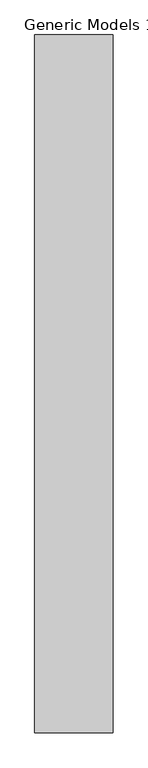
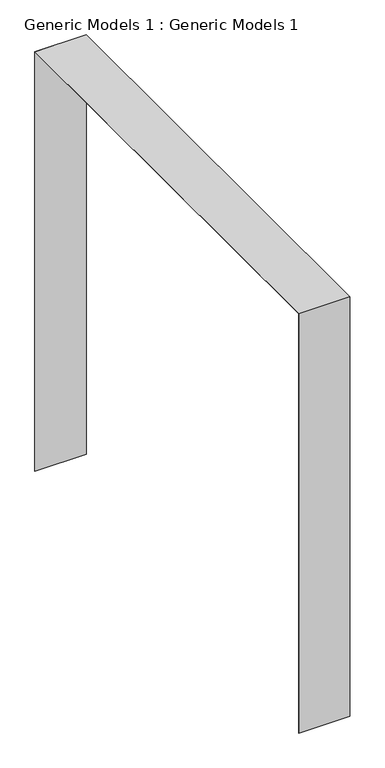
"""IFC4 building model written with IfcOpenShell, lengths in millimetres: proxy geometry, Generic Models 1 : Generic Models 1."""

import ifcopenshell
import ifcopenshell.guid

model = None  # the IFC model being written
_history = None  # IfcOwnerHistory: only IFC2X3 demands one
_inside = {}  # id of a spatial element -> (the spatial element, [elements in it])
_under = {}  # id of a project, library or spatial element -> (it, [spatial elements below it])
_declared = {}  # id of a project -> (the project, [libraries it declares])
_typed = {}  # id of a type object -> (the type object, [elements of that type])
_made_of = {}  # id of a material, layer set ... -> (it, [elements and type objects made of it])


def new_model(schema):
    """Start an empty IFC model of exactly this schema.

    Asked for "IFC4X3", IfcOpenShell would pick the latest addendum, in which some entities
    have other attributes; the version numbers below select the first issue.
    IFC2X3 requires an IfcOwnerHistory on every rooted entity: one is made here for all.
    """
    global model, _history
    if schema == "IFC4X3":
        model = ifcopenshell.file(schema_version=(4, 3, 0, 0))
    else:
        model = ifcopenshell.file(schema=schema)
    _inside.clear()
    _under.clear()
    _declared.clear()
    _typed.clear()
    _made_of.clear()
    _history = None
    if model.schema == "IFC2X3":
        org = make("IfcOrganization", Name="unknown")
        user = make(
            "IfcPersonAndOrganization",
            ThePerson=make("IfcPerson", FamilyName="unknown"),
            TheOrganization=org,
        )
        app = make(
            "IfcApplication",
            ApplicationDeveloper=org,
            Version="unknown",
            ApplicationFullName="unknown",
            ApplicationIdentifier="unknown",
        )
        _history = make(
            "IfcOwnerHistory",
            OwningUser=user,
            OwningApplication=app,
            ChangeAction="ADDED",
            CreationDate=0,
        )
    return model


def make(cls, **values):
    """One entity of the class cls with the attributes given. An attribute that is None is left unset."""
    return model.create_entity(
        cls, **{name: value for name, value in values.items() if value is not None}
    )


def rooted(cls, **values):
    """An entity with a GlobalId (a new one), such as an element, a storey or a relation."""
    return make(cls, GlobalId=ifcopenshell.guid.new(), OwnerHistory=_history, **values)


def si_unit(unit_type, name, prefix=None):
    """IfcSIUnit, for example si_unit("LENGTHUNIT", "METRE", prefix="MILLI")."""
    return make("IfcSIUnit", UnitType=unit_type, Prefix=prefix, Name=name)


def assignment(units):
    """IfcUnitAssignment: the units of a project."""
    return None if units is None else make("IfcUnitAssignment", Units=units)


def point(xyz):
    """IfcCartesianPoint."""
    return None if xyz is None else make("IfcCartesianPoint", Coordinates=xyz)


def direction(xyz):
    """IfcDirection."""
    return None if xyz is None else make("IfcDirection", DirectionRatios=xyz)


def frame(location, z_axis=None, x_axis=None):
    """IfcAxis2Placement3D, a coordinate frame: its origin and axes. An axis left out is left unset."""
    return make(
        "IfcAxis2Placement3D",
        Location=point(location),
        Axis=direction(z_axis),
        RefDirection=direction(x_axis),
    )


def origin():
    """The frame at (0, 0, 0) with its axes left unset."""
    return frame((0.0, 0.0, 0.0))


def place(relative_to, where):
    """IfcLocalPlacement: puts the frame where relative to a parent placement (None: the world)."""
    return make(
        "IfcLocalPlacement", PlacementRelTo=relative_to, RelativePlacement=where
    )


def context(
    kind, dimensions, precision=None, world=None, true_north=None, identifier=None
):
    """IfcGeometricRepresentationContext, for example the 3D "Model" context."""
    return make(
        "IfcGeometricRepresentationContext",
        ContextIdentifier=identifier,
        ContextType=kind,
        CoordinateSpaceDimension=dimensions,
        Precision=precision,
        WorldCoordinateSystem=world,
        TrueNorth=true_north,
    )


def project(units=None, contexts=None):
    """IfcProject with its units and contexts."""
    return rooted(
        "IfcProject",
        Name="project",
        RepresentationContexts=contexts,
        UnitsInContext=assignment(units),
    )


def spatial(cls, under=None, at=None, **own):
    """A site, building, storey or space (cls), placed at a placement, below another one or the project."""
    s = rooted(cls, ObjectPlacement=at, **own)
    if under is not None:
        _under.setdefault(under.id(), (under, []))[1].append(s)
    return s


def polyline(points):
    """IfcPolyline through the points."""
    return make("IfcPolyline", Points=[point(p) for p in points])


def outline(outer, holes=None, kind="AREA"):
    """IfcArbitraryClosedProfileDef: a profile drawn as a closed curve; with holes, ...WithVoids."""
    if holes is None:
        return make("IfcArbitraryClosedProfileDef", ProfileType=kind, OuterCurve=outer)
    return make(
        "IfcArbitraryProfileDefWithVoids",
        ProfileType=kind,
        OuterCurve=outer,
        InnerCurves=holes,
    )


def extrude(swept, where, along, depth):
    """IfcExtrudedAreaSolid: the profile swept, set in the frame where, extruded along a direction by depth."""
    return make(
        "IfcExtrudedAreaSolid",
        SweptArea=swept,
        Position=where,
        ExtrudedDirection=direction(along),
        Depth=depth,
    )


def shape(context_of_items, identifier, shape_type, items):
    """IfcShapeRepresentation: the items that make up one representation, for example the "Body"."""
    return make(
        "IfcShapeRepresentation",
        ContextOfItems=context_of_items,
        RepresentationIdentifier=identifier,
        RepresentationType=shape_type,
        Items=items,
    )


def source(mapping_origin, context_of_items, identifier, shape_type, items):
    """IfcRepresentationMap: a shape defined once, which mapped items show again and again."""
    return make(
        "IfcRepresentationMap",
        MappingOrigin=mapping_origin,
        MappedRepresentation=shape(context_of_items, identifier, shape_type, items),
    )


def transform(
    local_origin,
    x_axis=None,
    y_axis=None,
    z_axis=None,
    scale=None,
    scale2=None,
    scale3=None,
    uniform=True,
):
    """IfcCartesianTransformationOperator3D, or its non-uniform kind. x_axis, y_axis, z_axis: its Axis1, 2, 3."""
    if uniform:
        return make(
            "IfcCartesianTransformationOperator3D",
            Axis1=direction(x_axis),
            Axis2=direction(y_axis),
            LocalOrigin=point(local_origin),
            Scale=scale,
            Axis3=direction(z_axis),
        )
    return make(
        "IfcCartesianTransformationOperator3DnonUniform",
        Axis1=direction(x_axis),
        Axis2=direction(y_axis),
        LocalOrigin=point(local_origin),
        Scale=scale,
        Axis3=direction(z_axis),
        Scale2=scale2,
        Scale3=scale3,
    )


def mapped(mapping_source, mapping_target):
    """IfcMappedItem: shows the shape of a source again, moved by a transform."""
    return make(
        "IfcMappedItem", MappingSource=mapping_source, MappingTarget=mapping_target
    )


def made_of(thing, what):
    """Note that an element or type object is made of a material, layer set ...; save() writes the relation."""
    if what is not None:
        _made_of.setdefault(what.id(), (what, []))[1].append(thing)
    return thing


def element(
    cls,
    number,
    at=None,
    inside=None,
    cuts=None,
    type_object=None,
    material=None,
    context=None,
    identifier="Body",
    shape_type=None,
    held_by="IfcProductDefinitionShape",
    body=None,
    shapes=None,
    **own,
):
    """One element of the class cls, such as IfcWall. Its Tag is "e" and its number.

    at: its placement. inside: the storey or other place that contains it. cuts: it is an
    opening in that element (IfcRelVoidsElement). A single representation is given by context,
    identifier, shape_type and body (its items); several are given by shapes. held_by: the class
    of the entity that holds the representations. save() writes the other relations.
    """
    e = rooted(cls, Tag="e%d" % number, ObjectPlacement=at, **own)
    if body is not None:
        shapes = [shape(context, identifier, shape_type, body)]
    if shapes is not None:
        e.Representation = make(held_by, Representations=shapes)
    if inside is not None:
        _inside.setdefault(inside.id(), (inside, []))[1].append(e)
    if cuts is not None:
        rooted(
            "IfcRelVoidsElement", RelatingBuildingElement=cuts, RelatedOpeningElement=e
        )
    if type_object is not None:
        _typed.setdefault(type_object.id(), (type_object, []))[1].append(e)
    return made_of(e, material)


def aggregate(whole, parts):
    """IfcRelAggregates: a whole, such as a stair, and the parts it consists of."""
    return rooted("IfcRelAggregates", RelatingObject=whole, RelatedObjects=parts)


def save(model, path):
    """Write the relations noted so far, then the file.

    IfcRelAggregates (storeys below a building ...), IfcRelContainedInSpatialStructure (elements
    in a storey), IfcRelDefinesByType, IfcRelAssociatesMaterial and IfcRelDeclares: one each for
    every whole, place, type object, material and project.
    """
    for whole, parts in _under.values():
        aggregate(whole, parts)
    for where, things in _inside.values():
        rooted(
            "IfcRelContainedInSpatialStructure",
            RelatedElements=things,
            RelatingStructure=where,
        )
    for kind, things in _typed.values():
        rooted("IfcRelDefinesByType", RelatedObjects=things, RelatingType=kind)
    for what, things in _made_of.values():
        rooted("IfcRelAssociatesMaterial", RelatedObjects=things, RelatingMaterial=what)
    for by, libraries in _declared.values():
        rooted("IfcRelDeclares", RelatingContext=by, RelatedDefinitions=libraries)
    model.write(path)


def generic_models_1_generic_models_1_6dc33216(model_context):
    return source(origin(), model_context, "Body", "SweptSolid", [
        extrude(outline(polyline([(26552.7208589, 1749.9720055), (26551.7208589, 1749.9720055), (26551.7208589, 6598.9720055), (21553.7208589, 6598.9720055), (21553.7208589, 1749.9720055), (21552.7208589, 1749.9720055), (21552.7208589, 6599.9720055), (26552.7208589, 6599.9720055), (26552.7208589, 1749.9720055)])), frame((-935.0, 0.0, 0.0), z_axis=(1.0, 0.0, 0.0), x_axis=(0.0, 1.0, 0.0)), (0.0, 0.0, 1.0), 560.0),
    ])


if __name__ == "__main__":
    model = new_model("IFC4")
    model_context = context("Model", 3, world=origin())
    ifc_project = project(units=[si_unit("LENGTHUNIT", "METRE", prefix="MILLI")], contexts=[model_context])
    site = spatial("IfcSite", under=ifc_project)
    building = spatial("IfcBuilding", under=site)
    placement = place(None, origin())
    generic_models_1_generic_models_1_shape = generic_models_1_generic_models_1_6dc33216(model_context)
    element("IfcBuildingElementProxy", 1, Name="Generic Models 1 : Generic Models 1", ObjectType="Generic Models 1 : Generic Models 1", at=placement, inside=building, context=model_context, shape_type="MappedRepresentation", body=[
        mapped(generic_models_1_generic_models_1_shape, transform((0.0, 0.0, 0.0), x_axis=(1.0, 0.0, 0.0), y_axis=(0.0, 1.0, 0.0), z_axis=(0.0, 0.0, 1.0))),
    ])
    save(model, "model.ifc")
